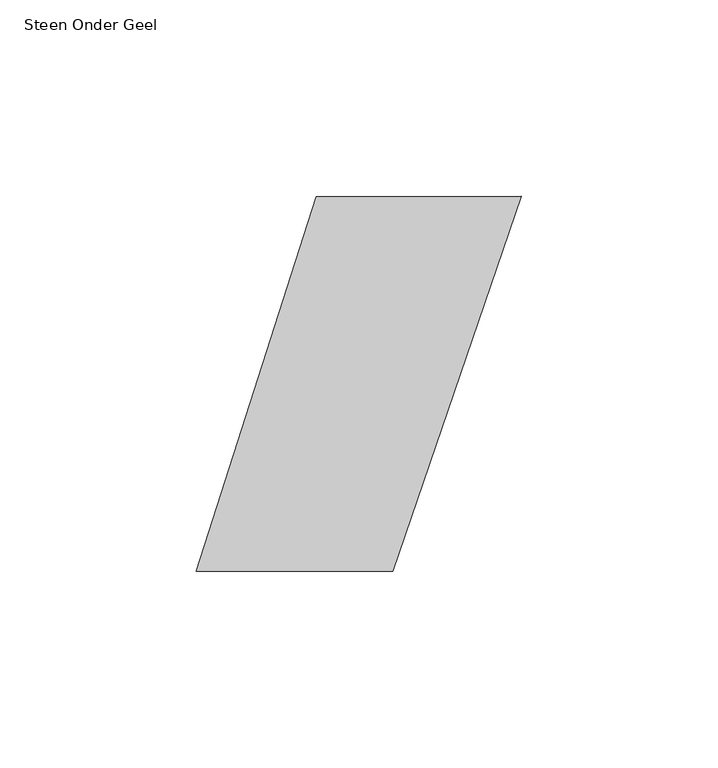
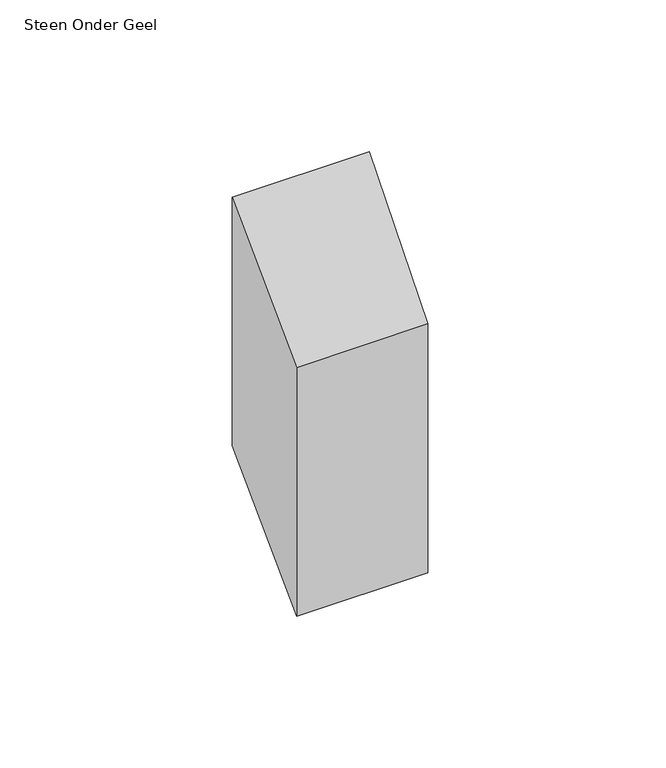
"""IFC4 building model written with IfcOpenShell, lengths in millimetres: proxy geometry, 00_GMA_steen_versie_4 : Steen Onder Geel."""

from ifc_helpers import new_model, si_unit, origin, origin_with_axes, place, context, project, spatial, polyline, outline, extrude, source, transform, mapped, element, save


def steen_onder_geel_74476426(model_context):
    return source(origin(), model_context, "Body", "SweptSolid", [
        extrude(outline(polyline([(116.0707694, 113.8841067), (83.4151391, 18.5589473), (33.41521, 18.4747478), (63.9435302, 113.7697957), (116.0707694, 113.8841067)])), origin_with_axes(), (0.0, 0.0, 1.0), 100.0),
    ])


if __name__ == "__main__":
    model = new_model("IFC4")
    model_context = context("Model", 3, world=origin())
    ifc_project = project(units=[si_unit("LENGTHUNIT", "METRE", prefix="MILLI")], contexts=[model_context])
    site = spatial("IfcSite", under=ifc_project)
    building = spatial("IfcBuilding", under=site)
    placement = place(None, origin())
    steen_onder_geel_shape = steen_onder_geel_74476426(model_context)
    element("IfcBuildingElementProxy", 1, Name="00_GMA_steen_versie_4 : Steen Onder Geel", ObjectType="00_GMA_steen_versie_4 : Steen Onder Geel", at=placement, inside=building, context=model_context, shape_type="MappedRepresentation", body=[
        mapped(steen_onder_geel_shape, transform((0.0, 0.0, 0.0), x_axis=(1.0, 0.0, 0.0), y_axis=(0.0, 1.0, 0.0), z_axis=(0.0, 0.0, 1.0))),
    ])
    save(model, "model.ifc")

# Revit data of these elements
# Type "00_GMA_steen_versie_4 : Steen Onder Geel"
#   StootVoegHalfBoven [instance default] = 5 mm
#   StootVoegHalf [instance default] = 5 mm
#   StootVoegBreedteOnder = 10 mm
#   StootVoegBreedteBoven = 10 mm
#   Steendikte = 100 mm
#   LintVoegOnderHalf = 0 mm
#   LintVoegOnder = 0 mm
#   LintVoegBovenHalf = 5 mm
#   LintVoegBoven = 10 mm
#   materiaal = 21_steen_geel
#   MateriaalVoeg = none
#   Default Elevation = 0
# Element 1 (IfcBuildingElementProxy, "00_GMA_steen_versie_4 : Steen Onder Geel")
#   Materials on its faces: "21_steen_geel"
# Materials
#   "21_steen_geel": class "Unassigned", colour RGB 202 202 0, transparency 0, Cost = 0
